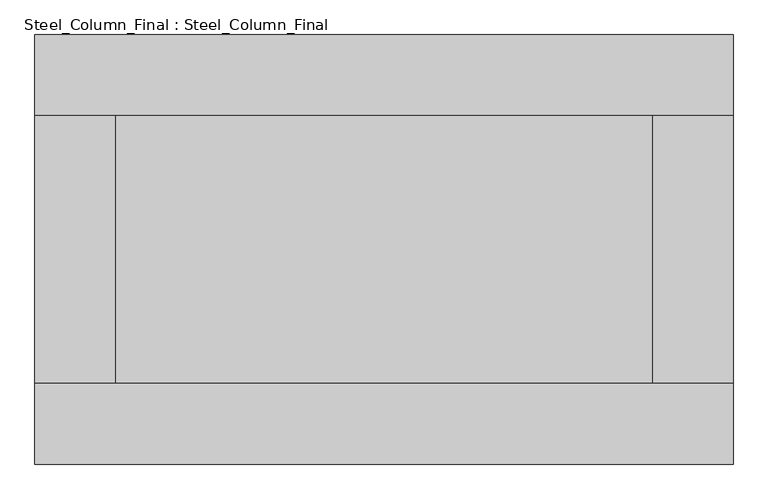
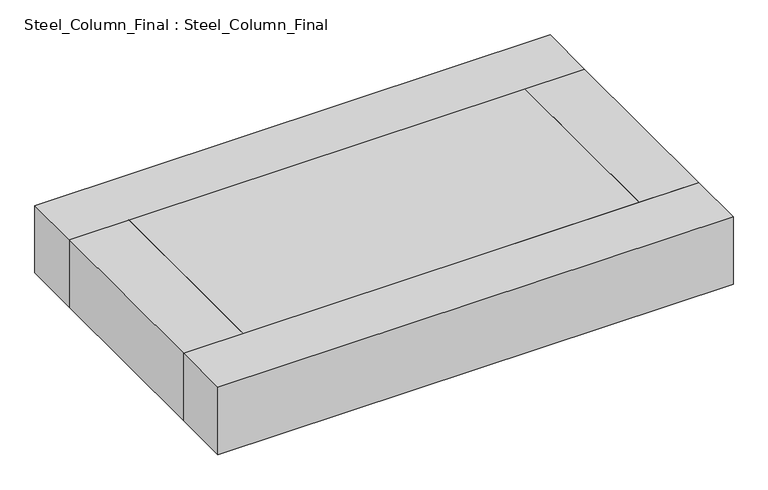
"""IFC4 building model written with IfcOpenShell, lengths in millimetres: proxy geometry, Steel_Column_Final : Steel_Column_Final."""

import ifcopenshell
import ifcopenshell.guid

model = None  # the IFC model being written
_history = None  # IfcOwnerHistory: only IFC2X3 demands one
_inside = {}  # id of a spatial element -> (the spatial element, [elements in it])
_under = {}  # id of a project, library or spatial element -> (it, [spatial elements below it])
_declared = {}  # id of a project -> (the project, [libraries it declares])
_typed = {}  # id of a type object -> (the type object, [elements of that type])
_made_of = {}  # id of a material, layer set ... -> (it, [elements and type objects made of it])


def new_model(schema):
    """Start an empty IFC model of exactly this schema.

    Asked for "IFC4X3", IfcOpenShell would pick the latest addendum, in which some entities
    have other attributes; the version numbers below select the first issue.
    IFC2X3 requires an IfcOwnerHistory on every rooted entity: one is made here for all.
    """
    global model, _history
    if schema == "IFC4X3":
        model = ifcopenshell.file(schema_version=(4, 3, 0, 0))
    else:
        model = ifcopenshell.file(schema=schema)
    _inside.clear()
    _under.clear()
    _declared.clear()
    _typed.clear()
    _made_of.clear()
    _history = None
    if model.schema == "IFC2X3":
        org = make("IfcOrganization", Name="unknown")
        user = make(
            "IfcPersonAndOrganization",
            ThePerson=make("IfcPerson", FamilyName="unknown"),
            TheOrganization=org,
        )
        app = make(
            "IfcApplication",
            ApplicationDeveloper=org,
            Version="unknown",
            ApplicationFullName="unknown",
            ApplicationIdentifier="unknown",
        )
        _history = make(
            "IfcOwnerHistory",
            OwningUser=user,
            OwningApplication=app,
            ChangeAction="ADDED",
            CreationDate=0,
        )
    return model


def make(cls, **values):
    """One entity of the class cls with the attributes given. An attribute that is None is left unset."""
    return model.create_entity(
        cls, **{name: value for name, value in values.items() if value is not None}
    )


def rooted(cls, **values):
    """An entity with a GlobalId (a new one), such as an element, a storey or a relation."""
    return make(cls, GlobalId=ifcopenshell.guid.new(), OwnerHistory=_history, **values)


def si_unit(unit_type, name, prefix=None):
    """IfcSIUnit, for example si_unit("LENGTHUNIT", "METRE", prefix="MILLI")."""
    return make("IfcSIUnit", UnitType=unit_type, Prefix=prefix, Name=name)


def assignment(units):
    """IfcUnitAssignment: the units of a project."""
    return None if units is None else make("IfcUnitAssignment", Units=units)


def point(xyz):
    """IfcCartesianPoint."""
    return None if xyz is None else make("IfcCartesianPoint", Coordinates=xyz)


def direction(xyz):
    """IfcDirection."""
    return None if xyz is None else make("IfcDirection", DirectionRatios=xyz)


def frame(location, z_axis=None, x_axis=None):
    """IfcAxis2Placement3D, a coordinate frame: its origin and axes. An axis left out is left unset."""
    return make(
        "IfcAxis2Placement3D",
        Location=point(location),
        Axis=direction(z_axis),
        RefDirection=direction(x_axis),
    )


def origin():
    """The frame at (0, 0, 0) with its axes left unset."""
    return frame((0.0, 0.0, 0.0))


def place(relative_to, where):
    """IfcLocalPlacement: puts the frame where relative to a parent placement (None: the world)."""
    return make(
        "IfcLocalPlacement", PlacementRelTo=relative_to, RelativePlacement=where
    )


def context(
    kind, dimensions, precision=None, world=None, true_north=None, identifier=None
):
    """IfcGeometricRepresentationContext, for example the 3D "Model" context."""
    return make(
        "IfcGeometricRepresentationContext",
        ContextIdentifier=identifier,
        ContextType=kind,
        CoordinateSpaceDimension=dimensions,
        Precision=precision,
        WorldCoordinateSystem=world,
        TrueNorth=true_north,
    )


def project(units=None, contexts=None):
    """IfcProject with its units and contexts."""
    return rooted(
        "IfcProject",
        Name="project",
        RepresentationContexts=contexts,
        UnitsInContext=assignment(units),
    )


def spatial(cls, under=None, at=None, **own):
    """A site, building, storey or space (cls), placed at a placement, below another one or the project."""
    s = rooted(cls, ObjectPlacement=at, **own)
    if under is not None:
        _under.setdefault(under.id(), (under, []))[1].append(s)
    return s


def polyline(points):
    """IfcPolyline through the points."""
    return make("IfcPolyline", Points=[point(p) for p in points])


def outline(outer, holes=None, kind="AREA"):
    """IfcArbitraryClosedProfileDef: a profile drawn as a closed curve; with holes, ...WithVoids."""
    if holes is None:
        return make("IfcArbitraryClosedProfileDef", ProfileType=kind, OuterCurve=outer)
    return make(
        "IfcArbitraryProfileDefWithVoids",
        ProfileType=kind,
        OuterCurve=outer,
        InnerCurves=holes,
    )


def extrude(swept, where, along, depth):
    """IfcExtrudedAreaSolid: the profile swept, set in the frame where, extruded along a direction by depth."""
    return make(
        "IfcExtrudedAreaSolid",
        SweptArea=swept,
        Position=where,
        ExtrudedDirection=direction(along),
        Depth=depth,
    )


def shape(context_of_items, identifier, shape_type, items):
    """IfcShapeRepresentation: the items that make up one representation, for example the "Body"."""
    return make(
        "IfcShapeRepresentation",
        ContextOfItems=context_of_items,
        RepresentationIdentifier=identifier,
        RepresentationType=shape_type,
        Items=items,
    )


def source(mapping_origin, context_of_items, identifier, shape_type, items):
    """IfcRepresentationMap: a shape defined once, which mapped items show again and again."""
    return make(
        "IfcRepresentationMap",
        MappingOrigin=mapping_origin,
        MappedRepresentation=shape(context_of_items, identifier, shape_type, items),
    )


def transform(
    local_origin,
    x_axis=None,
    y_axis=None,
    z_axis=None,
    scale=None,
    scale2=None,
    scale3=None,
    uniform=True,
):
    """IfcCartesianTransformationOperator3D, or its non-uniform kind. x_axis, y_axis, z_axis: its Axis1, 2, 3."""
    if uniform:
        return make(
            "IfcCartesianTransformationOperator3D",
            Axis1=direction(x_axis),
            Axis2=direction(y_axis),
            LocalOrigin=point(local_origin),
            Scale=scale,
            Axis3=direction(z_axis),
        )
    return make(
        "IfcCartesianTransformationOperator3DnonUniform",
        Axis1=direction(x_axis),
        Axis2=direction(y_axis),
        LocalOrigin=point(local_origin),
        Scale=scale,
        Axis3=direction(z_axis),
        Scale2=scale2,
        Scale3=scale3,
    )


def mapped(mapping_source, mapping_target):
    """IfcMappedItem: shows the shape of a source again, moved by a transform."""
    return make(
        "IfcMappedItem", MappingSource=mapping_source, MappingTarget=mapping_target
    )


def made_of(thing, what):
    """Note that an element or type object is made of a material, layer set ...; save() writes the relation."""
    if what is not None:
        _made_of.setdefault(what.id(), (what, []))[1].append(thing)
    return thing


def element(
    cls,
    number,
    at=None,
    inside=None,
    cuts=None,
    type_object=None,
    material=None,
    context=None,
    identifier="Body",
    shape_type=None,
    held_by="IfcProductDefinitionShape",
    body=None,
    shapes=None,
    **own,
):
    """One element of the class cls, such as IfcWall. Its Tag is "e" and its number.

    at: its placement. inside: the storey or other place that contains it. cuts: it is an
    opening in that element (IfcRelVoidsElement). A single representation is given by context,
    identifier, shape_type and body (its items); several are given by shapes. held_by: the class
    of the entity that holds the representations. save() writes the other relations.
    """
    e = rooted(cls, Tag="e%d" % number, ObjectPlacement=at, **own)
    if body is not None:
        shapes = [shape(context, identifier, shape_type, body)]
    if shapes is not None:
        e.Representation = make(held_by, Representations=shapes)
    if inside is not None:
        _inside.setdefault(inside.id(), (inside, []))[1].append(e)
    if cuts is not None:
        rooted(
            "IfcRelVoidsElement", RelatingBuildingElement=cuts, RelatedOpeningElement=e
        )
    if type_object is not None:
        _typed.setdefault(type_object.id(), (type_object, []))[1].append(e)
    return made_of(e, material)


def aggregate(whole, parts):
    """IfcRelAggregates: a whole, such as a stair, and the parts it consists of."""
    return rooted("IfcRelAggregates", RelatingObject=whole, RelatedObjects=parts)


def save(model, path):
    """Write the relations noted so far, then the file.

    IfcRelAggregates (storeys below a building ...), IfcRelContainedInSpatialStructure (elements
    in a storey), IfcRelDefinesByType, IfcRelAssociatesMaterial and IfcRelDeclares: one each for
    every whole, place, type object, material and project.
    """
    for whole, parts in _under.values():
        aggregate(whole, parts)
    for where, things in _inside.values():
        rooted(
            "IfcRelContainedInSpatialStructure",
            RelatedElements=things,
            RelatingStructure=where,
        )
    for kind, things in _typed.values():
        rooted("IfcRelDefinesByType", RelatedObjects=things, RelatingType=kind)
    for what, things in _made_of.values():
        rooted("IfcRelAssociatesMaterial", RelatedObjects=things, RelatingMaterial=what)
    for by, libraries in _declared.values():
        rooted("IfcRelDeclares", RelatingContext=by, RelatedDefinitions=libraries)
    model.write(path)


def steel_column_final_steel_column_final_90d007b7(model_context):
    return source(origin(), model_context, "Body", "SweptSolid", [
        extrude(outline(polyline([(6500.0, 2500.0), (-6500.0, 2500.0), (-6500.0, 4000.0), (6500.0, 4000.0), (6500.0, 2500.0)])), frame((0.0, 0.0, 8880.0), z_axis=(0.0, 0.0, 1.0), x_axis=(1.0, 0.0, 0.0)), (0.0, 0.0, 1.0), 1800.0),
        extrude(outline(polyline([(-6500.0, -2500.0), (6500.0, -2500.0), (6500.0, -4000.0), (-6500.0, -4000.0), (-6500.0, -2500.0)])), frame((0.0, 0.0, 8880.0), z_axis=(0.0, 0.0, 1.0), x_axis=(1.0, 0.0, 0.0)), (0.0, 0.0, 1.0), 1800.0),
        extrude(outline(polyline([(5000.0, -2500.0), (5000.0, 2500.0), (6500.0, 2500.0), (6500.0, -2500.0), (5000.0, -2500.0)])), frame((0.0, 0.0, 8880.0), z_axis=(0.0, 0.0, 1.0), x_axis=(1.0, 0.0, 0.0)), (0.0, 0.0, 1.0), 1800.0),
        extrude(outline(polyline([(-5000.0, 2500.0), (-5000.0, -2500.0), (-6500.0, -2500.0), (-6500.0, 2500.0), (-5000.0, 2500.0)])), frame((0.0, 0.0, 8880.0), z_axis=(0.0, 0.0, 1.0), x_axis=(1.0, 0.0, 0.0)), (0.0, 0.0, 1.0), 1800.0),
        extrude(outline(polyline([(-5000.0, -2500.0), (-5000.0, 2500.0), (5000.0, 2500.0), (5000.0, -2500.0), (-5000.0, -2500.0)])), frame((0.0, 0.0, 8880.0), z_axis=(0.0, 0.0, 1.0), x_axis=(1.0, 0.0, 0.0)), (0.0, 0.0, 1.0), 1800.0),
    ])


if __name__ == "__main__":
    model = new_model("IFC4")
    model_context = context("Model", 3, world=origin())
    ifc_project = project(units=[si_unit("LENGTHUNIT", "METRE", prefix="MILLI")], contexts=[model_context])
    site = spatial("IfcSite", under=ifc_project)
    building = spatial("IfcBuilding", under=site)
    placement = place(None, origin())
    steel_column_final_steel_column_final_shape = steel_column_final_steel_column_final_90d007b7(model_context)
    element("IfcBuildingElementProxy", 1, Name="Steel_Column_Final : Steel_Column_Final", ObjectType="Steel_Column_Final : Steel_Column_Final", at=placement, inside=building, context=model_context, shape_type="MappedRepresentation", body=[
        mapped(steel_column_final_steel_column_final_shape, transform((0.0, 0.0, 0.0), x_axis=(1.0, 0.0, 0.0), y_axis=(0.0, 1.0, 0.0), z_axis=(0.0, 0.0, 1.0))),
    ])
    save(model, "model.ifc")

# Revit data of these elements
# Type "Steel_Column_Final : Steel_Column_Final"
#   Top Width [instance default] = 5000 mm
#   Top Length = 10000 mm
#   Length = 21000 mm
#   Height [instance default] = 50000 mm
#   Bottom Width [instance default] = 5000 mm
#   Default Elevation = 0
# Element 1 (IfcBuildingElementProxy, "Steel_Column_Final : Steel_Column_Final")
#   Height = 8880 mm
